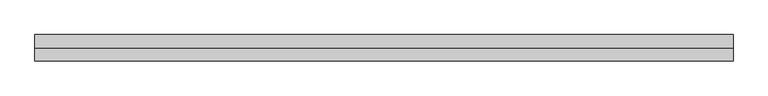
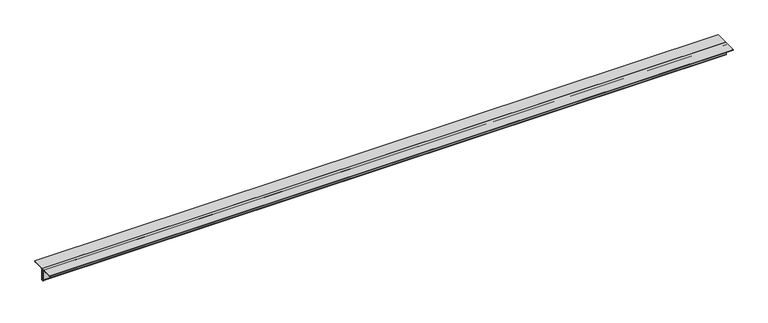
"""IFC4 building model written with IfcOpenShell, lengths in millimetres: member geometry, 0123_Steel Framing_2Ls-KSD3502 : H_SB_AR_S03_2Ls-130x130x12_HBR4."""

from ifc_helpers import new_model, si_unit, point, frame, frame_2d, origin, place, context, project, spatial, polyline, circle_curve, trimmed, segment, composite_curve, outline, extrude, source, transform, mapped, element, save


def member_85476d18(model_context):
    return source(origin(), model_context, "Body", "SweptSolid", [
        extrude(outline(composite_curve([segment(polyline([(0.0, 36.4), (130.0, 36.4)]), True, "CONTINUOUS"), segment(trimmed(circle_curve(frame_2d((118.0, 36.4)), 12.0), [point((130.0, 36.4))], [point((118.0, 24.4))], False, "CARTESIAN"), True, "CONTINUOUS"), segment(polyline([(118.0, 24.4), (24.0, 24.4)]), True, "CONTINUOUS"), segment(trimmed(circle_curve(frame_2d((24.0, 12.4)), 12.0), [point((24.0, 24.4))], [point((12.0, 12.4))], True, "CARTESIAN"), True, "CONTINUOUS"), segment(polyline([(12.0, 12.4), (12.0, -81.6)]), True, "CONTINUOUS"), segment(trimmed(circle_curve(frame_2d((0.0, -81.6)), 12.0), [point((12.0, -81.6))], [point((0.0, -93.6))], False, "CARTESIAN"), True, "CONTINUOUS"), segment(polyline([(0.0, -93.6), (0.0, 36.4)]), True, "CONTINUOUS")], self_intersect=False)), frame((-3436.1943157, 0.0, 0.0), z_axis=(1.0, 0.0, 0.0), x_axis=(0.0, 1.0, 0.0)), (0.0, 0.0, 1.0), 6850.1941634),
        extrude(outline(composite_curve([segment(polyline([(0.0, 36.4), (0.0, -93.6)]), True, "CONTINUOUS"), segment(trimmed(circle_curve(frame_2d((0.0, -81.6)), 12.0), [point((0.0, -93.6))], [point((-12.0, -81.6))], False, "CARTESIAN"), True, "CONTINUOUS"), segment(polyline([(-12.0, -81.6), (-12.0, 12.4)]), True, "CONTINUOUS"), segment(trimmed(circle_curve(frame_2d((-24.0, 12.4)), 12.0), [point((-12.0, 12.4))], [point((-24.0, 24.4))], True, "CARTESIAN"), True, "CONTINUOUS"), segment(polyline([(-24.0, 24.4), (-118.0, 24.4)]), True, "CONTINUOUS"), segment(trimmed(circle_curve(frame_2d((-118.0, 36.4)), 12.0), [point((-118.0, 24.4))], [point((-130.0, 36.4))], False, "CARTESIAN"), True, "CONTINUOUS"), segment(polyline([(-130.0, 36.4), (0.0, 36.4)]), True, "CONTINUOUS")], self_intersect=False)), frame((-3436.1943157, 0.0, 0.0), z_axis=(1.0, 0.0, 0.0), x_axis=(0.0, 1.0, 0.0)), (0.0, 0.0, 1.0), 6850.1941634),
    ])


if __name__ == "__main__":
    model = new_model("IFC4")
    model_context = context("Model", 3, world=origin())
    ifc_project = project(units=[si_unit("LENGTHUNIT", "METRE", prefix="MILLI")], contexts=[model_context])
    site = spatial("IfcSite", under=ifc_project)
    building = spatial("IfcBuilding", under=site)
    placement = place(None, origin())
    member_shape = member_85476d18(model_context)
    element("IfcMember", 1, ObjectType="0123_Steel Framing_2Ls-KSD3502 : H_SB_AR_S03_2Ls-130x130x12_HBR4", at=placement, inside=building, context=model_context, shape_type="MappedRepresentation", body=[
        mapped(member_shape, transform((0.0, 0.0, 0.0), x_axis=(1.0, 0.0, 0.0), y_axis=(0.0, 1.0, 0.0), z_axis=(0.0, 0.0, 1.0))),
    ])
    save(model, "model.ifc")

# Revit data of these elements
# Type "0123_Steel Framing_2Ls-KSD3502 : H_SB_AR_S03_2Ls-130x130x12_HBR4"
#   Assembly Code = "B10"
#   Legs = "SLBB"
#   W = 8.97
#   Perimeter = 1.04 m²/m
#   Nominal Weight = 46.80 kgf/m
#   Length [instance default] = 1000 mm
#   Space = 0 mm
#   b = 130 mm
#   d = 130 mm
#   t = 12 mm
#   y = 36.4 mm
#   A = 0.005952 m²
#   Structural Material [instance default] = Steel ASTM A36
# Element 1 (IfcMember, "0123_Steel Framing_2Ls-KSD3502 : H_SB_AR_S03_2Ls-130x130x12_HBR4")
#   Structural Material = Steel, 45-345
#   Materials on its faces: "Steel, 45-345"
# Materials
#   "Steel ASTM A36": class "Metal", colour RGB 199 199 199, transparency 0, Description = "Structural steel, ASTM A36 Grade B, mill finish", Cost = 0
#   "Steel, 45-345": class "Metal", colour RGB 189 187 185, transparency 0, Description = "Steel 345 MPa", Cost = 0
